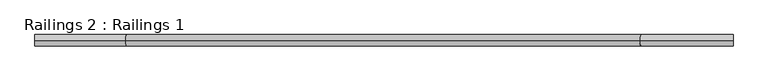
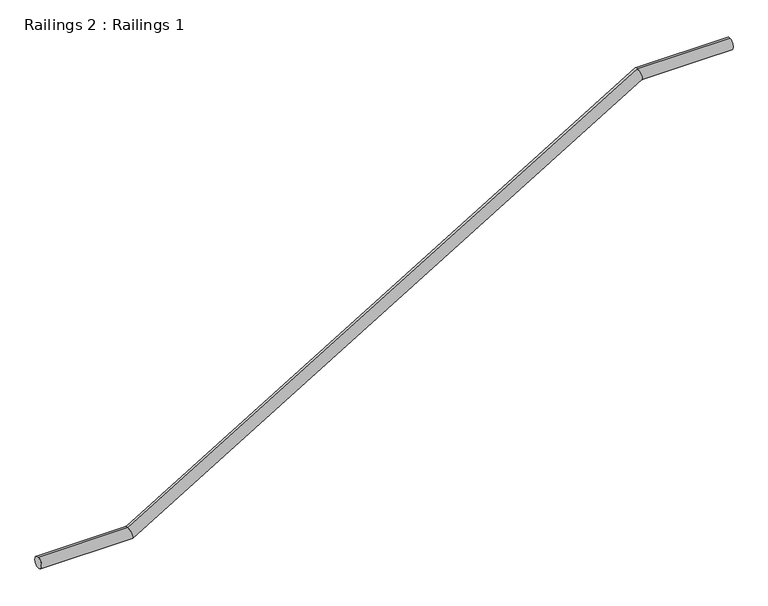
"""IFC4 building model written with IfcOpenShell, lengths in millimetres: railing geometry, Railings 2 : Railings 1."""

from ifc_helpers import new_model, si_unit, frame, origin, place, context, project, spatial, circle_curve, ellipse_curve, source, transform, mapped, element, save
from ifc_brep_helpers import plane_surface, cylinder_surface, advanced_brep


def railings_2_railings_1_6d3c6824(model_context):
    return source(origin(), model_context, "Body", "AdvancedBrep", [
        advanced_brep(
        [(25211.656657, 25875.3156612, 266268.2), (25211.656657, 25875.3156612, 266230.1), (27529.2868456, 25875.3156612, 267296.9), (27529.2868456, 25875.3156612, 267258.8), (25511.162987, 25875.3156612, 266268.2), (25521.7503269, 25875.3156612, 266230.1), (27219.1931757, 25875.3156612, 267296.9), (27229.7805156, 25875.3156612, 267258.8)],
        [
            (0, 1, circle_curve(frame((25211.656657, 25875.3156612, 266249.15), z_axis=(-1.0, 0.0, 0.0), x_axis=(0.0, 0.0, -1.0)), 19.05)),
            (1, 0, circle_curve(frame((25211.656657, 25875.3156612, 266249.15), z_axis=(-1.0, 0.0, 0.0), x_axis=(0.0, 0.0, -1.0)), 19.05)),
            (2, 3, circle_curve(frame((27529.2868456, 25875.3156612, 267277.85), z_axis=(1.0, 0.0, 0.0), x_axis=(0.0, 0.0, -1.0)), 19.05)),
            (3, 2, circle_curve(frame((27529.2868456, 25875.3156612, 267277.85), z_axis=(1.0, 0.0, 0.0), x_axis=(0.0, 0.0, -1.0)), 19.05)),
            (0, 4),
            (4, 5, ellipse_curve(frame((25516.456657, 25875.3156612, 266249.15), z_axis=(-0.9634917766912388, 0.0, -0.26773792456123974), x_axis=(-0.2677379245612396, 0.0, 0.9634917766912388)), 19.7718346, 19.05)),
            (5, 1),
            (5, 4, ellipse_curve(frame((25516.456657, 25875.3156612, 266249.15), z_axis=(-0.9634917766912388, 0.0, -0.26773792456123974), x_axis=(-0.2677379245612396, 0.0, 0.9634917766912388)), 19.7718346, 19.05)),
            (4, 6),
            (6, 7, ellipse_curve(frame((27224.4868456, 25875.3156612, 267277.85), z_axis=(-0.9634917766912388, 0.0, -0.26773792456123974), x_axis=(0.2677379245612396, 0.0, -0.9634917766912388)), 19.7718346, 19.05)),
            (7, 5),
            (7, 6, ellipse_curve(frame((27224.4868456, 25875.3156612, 267277.85), z_axis=(-0.9634917766912388, 0.0, -0.26773792456123974), x_axis=(0.2677379245612396, 0.0, -0.9634917766912388)), 19.7718346, 19.05)),
            (6, 2),
            (3, 7),
        ],
        [
            plane_surface(frame((25211.656657, 25856.2656612, 266249.15), z_axis=(-1.0, 0.0, 0.0), x_axis=(0.0, -1.0, 0.0))),
            plane_surface(frame((27529.2868456, 25856.2656612, 267277.85), z_axis=(1.0, 0.0, 0.0), x_axis=(0.0, -1.0, 0.0))),
            cylinder_surface(frame((25211.656657, 25875.3156612, 266249.15), z_axis=(-1.0, 0.0, 0.0), x_axis=(0.0, 0.0, -1.0)), 19.05),
            cylinder_surface(frame((25516.456657, 25875.3156612, 266249.15), z_axis=(-0.8566328075032799, 0.0, -0.5159265772462674), x_axis=(0.5159265772462674, 0.0, -0.8566328075032799)), 19.05),
            cylinder_surface(frame((27224.4868456, 25875.3156612, 267277.85), z_axis=(-1.0, 0.0, 0.0), x_axis=(0.0, 0.0, -1.0)), 19.05),
        ],
        [
            (0, [[1, 2]]),
            (1, [[3, 4]]),
            (2, [[-1, 5, 6, 7]]),
            (2, [[-2, -7, 8, -5]]),
            (3, [[-6, 9, 10, 11]]),
            (3, [[-8, -11, 12, -9]]),
            (4, [[-10, 13, -4, 14]]),
            (4, [[-12, -14, -3, -13]]),
        ],
    ),
    ])


if __name__ == "__main__":
    model = new_model("IFC4")
    model_context = context("Model", 3, world=origin())
    ifc_project = project(units=[si_unit("LENGTHUNIT", "METRE", prefix="MILLI")], contexts=[model_context])
    site = spatial("IfcSite", under=ifc_project)
    building = spatial("IfcBuilding", under=site)
    placement = place(None, origin())
    railings_2_railings_1_shape = railings_2_railings_1_6d3c6824(model_context)
    element("IfcRailing", 1, ObjectType="Railings 2 : Railings 1", at=placement, inside=building, context=model_context, shape_type="MappedRepresentation", body=[
        mapped(railings_2_railings_1_shape, transform((0.0, 0.0, 0.0), x_axis=(1.0, 0.0, 0.0), y_axis=(0.0, 1.0, 0.0), z_axis=(0.0, 0.0, 1.0))),
    ])
    save(model, "model.ifc")

# Revit data of these elements
# Element 1 (IfcRailing, "Railings 2 : Railings 1")
#   Materials on its faces: "ALUM. RAILING"
# Materials
#   "ALUM. RAILING": class "Generic", colour RGB 255 255 255, transparency 0, Cost = 0
